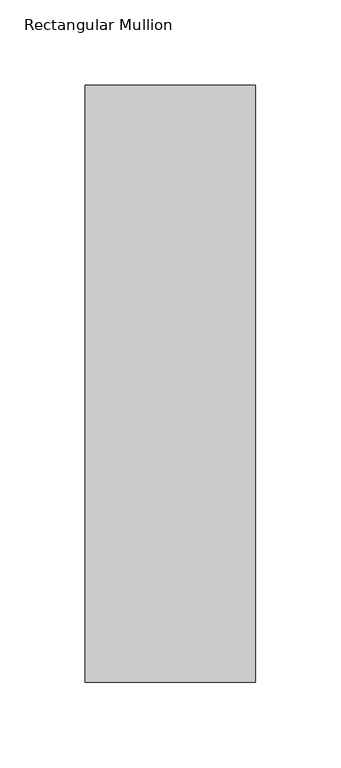
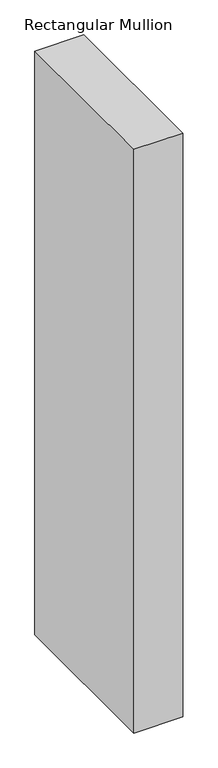
"""IFC4 building model written with IfcOpenShell, lengths in millimetres: member geometry, Rectangular Mullion : WWm-100x350-100mmOffset."""

from ifc_helpers import new_model, si_unit, frame, origin, place, context, project, spatial, polyline, outline, extrude, source, transform, mapped, element, save


def rectangular_mullion_d02dee49(model_context):
    return source(origin(), model_context, "Body", "SweptSolid", [
        extrude(outline(polyline([(0.0, 175.0), (0.0, -175.0), (-100.0, -175.0), (-100.0, 175.0), (0.0, 175.0)])), frame((0.0, 0.0, -1260.0), z_axis=(0.0, 0.0, 1.0), x_axis=(1.0, 0.0, 0.0)), (0.0, 0.0, 1.0), 1260.0),
    ])


if __name__ == "__main__":
    model = new_model("IFC4")
    model_context = context("Model", 3, world=origin())
    ifc_project = project(units=[si_unit("LENGTHUNIT", "METRE", prefix="MILLI")], contexts=[model_context])
    site = spatial("IfcSite", under=ifc_project)
    building = spatial("IfcBuilding", under=site)
    placement = place(None, origin())
    rectangular_mullion_shape = rectangular_mullion_d02dee49(model_context)
    element("IfcMember", 1, ObjectType="Rectangular Mullion : WWm-100x350-100mmOffset", at=placement, inside=building, context=model_context, shape_type="MappedRepresentation", body=[
        mapped(rectangular_mullion_shape, transform((0.0, 0.0, 0.0), x_axis=(1.0, 0.0, 0.0), y_axis=(0.0, 1.0, 0.0), z_axis=(0.0, 0.0, 1.0))),
    ])
    save(model, "model.ifc")

# Revit data of these elements
# Type "Rectangular Mullion : WWm-100x350-100mmOffset"
#   built-in parameter 1007304 = 1.14829 (stored number, unit not read)
#   built-in parameter 1007301 = 0.164042 (stored number, unit not read)
#   built-in parameter 1007300 = 0.164042 (stored number, unit not read)
# Element 1 (IfcMember, "Rectangular Mullion : WWm-100x350-100mmOffset")
#   Materials on its faces: "WW-EC-RGB-Mullion"
# Materials
#   "WW-EC-RGB-Mullion": class "Generic", colour RGB 255 255 255, transparency 0, Comments = "If region requests black mullions, switch asset color to RGB 25-25-25", Description = "Generic Color", Cost = 0
